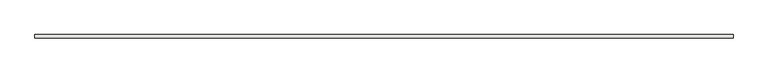
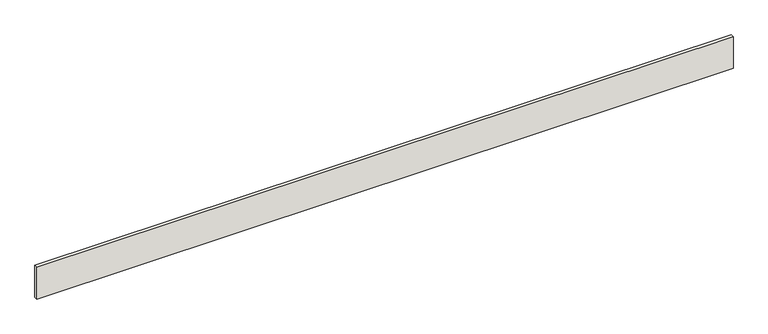
"""IFC4 building model written with IfcOpenShell, lengths in millimetres: wall geometry, Holzwand."""

from ifc_helpers import new_model, si_unit, origin, origin_with_axes, place, context, project, spatial, polyline, outline, extrude, source, transform, mapped, element, save


def wall_61fe101a(model_context):
    return source(origin(), model_context, "Body", "SweptSolid", [
        extrude(outline(polyline([(20802.8619019, 100.0), (20802.8619019, 0.0), (0.0, 0.0), (0.0, 100.0), (20802.8619019, 100.0)])), origin_with_axes(), (0.0, 0.0, 1.0), 1000.0),
    ])


if __name__ == "__main__":
    model = new_model("IFC4")
    model_context = context("Model", 3, world=origin())
    ifc_project = project(units=[si_unit("LENGTHUNIT", "METRE", prefix="MILLI")], contexts=[model_context])
    site = spatial("IfcSite", under=ifc_project)
    building = spatial("IfcBuilding", under=site)
    placement = place(None, origin())
    wall_shape = wall_61fe101a(model_context)
    element("IfcWall", 1, ObjectType="Holzwand", at=placement, inside=building, context=model_context, shape_type="MappedRepresentation", body=[
        mapped(wall_shape, transform((0.0, 0.0, 0.0), x_axis=(1.0, 0.0, 0.0), y_axis=(0.0, 1.0, 0.0), z_axis=(0.0, 0.0, 1.0))),
    ])
    save(model, "model.ifc")

# Revit data of these elements
# Element 1 (IfcWall, "Holzwand")
#   Materials on its faces: "pv - panel anthrazit"
# Materials
#   "pv - panel anthrazit": class "Unassigned", colour RGB 128 128 128, transparency 0
